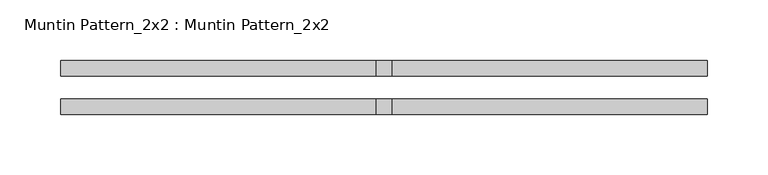
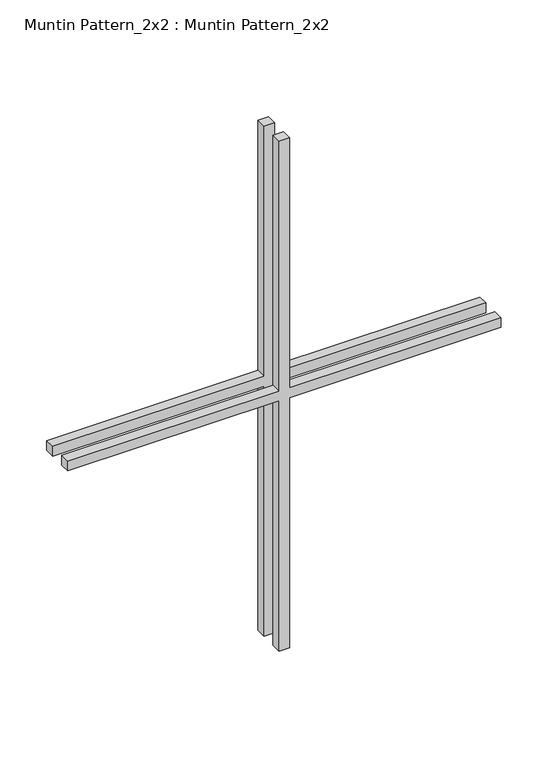
"""IFC4 building model written with IfcOpenShell, lengths in millimetres: proxy geometry, Muntin Pattern_2x2 : Muntin Pattern_2x2."""

from ifc_helpers import new_model, si_unit, frame, origin, place, context, project, spatial, polyline, outline, extrude, source, transform, mapped, element, save


def muntin_pattern_2x2_muntin_pattern_2x2_f10761d2(model_context):
    return source(origin(), model_context, "Body", "SweptSolid", [
        extrude(outline(polyline([(338.1375, -6.35), (338.1375, -266.7), (325.4375, -266.7), (325.4375, -6.35), (0.0, -6.35), (0.0, 6.35), (325.4375, 6.35), (325.4375, 266.7), (338.1375, 266.7), (338.1375, 6.35), (663.575, 6.35), (663.575, -6.35), (338.1375, -6.35)])), frame((0.0, -22.225, 0.0), z_axis=(0.0, 1.0, 0.0), x_axis=(0.0, 0.0, 1.0)), (0.0, 0.0, 1.0), 12.7),
        extrude(outline(polyline([(338.1375, -6.35), (338.1375, -266.7), (325.4375, -266.7), (325.4375, -6.35), (0.0, -6.35), (0.0, 6.35), (325.4375, 6.35), (325.4375, 266.7), (338.1375, 266.7), (338.1375, 6.35), (663.575, 6.35), (663.575, -6.35), (338.1375, -6.35)])), frame((0.0, 9.525, 0.0), z_axis=(0.0, 1.0, 0.0), x_axis=(0.0, 0.0, 1.0)), (0.0, 0.0, 1.0), 12.7),
    ])


if __name__ == "__main__":
    model = new_model("IFC4")
    model_context = context("Model", 3, world=origin())
    ifc_project = project(units=[si_unit("LENGTHUNIT", "METRE", prefix="MILLI")], contexts=[model_context])
    site = spatial("IfcSite", under=ifc_project)
    building = spatial("IfcBuilding", under=site)
    placement = place(None, origin())
    muntin_pattern_2x2_muntin_pattern_2x2_shape = muntin_pattern_2x2_muntin_pattern_2x2_f10761d2(model_context)
    element("IfcBuildingElementProxy", 1, Name="Muntin Pattern_2x2 : Muntin Pattern_2x2", ObjectType="Muntin Pattern_2x2 : Muntin Pattern_2x2", at=placement, inside=building, context=model_context, shape_type="MappedRepresentation", body=[
        mapped(muntin_pattern_2x2_muntin_pattern_2x2_shape, transform((0.0, 0.0, 0.0), x_axis=(1.0, 0.0, 0.0), y_axis=(0.0, 1.0, 0.0), z_axis=(0.0, 0.0, 1.0))),
    ])
    save(model, "model.ifc")

# Revit data of these elements
# Type "Muntin Pattern_2x2 : Muntin Pattern_2x2"
#   Width [instance default] = 4' - 0"
#   Thickness = 0' - 0 1/2"
#   Height [instance default] = 4' - 0"
#   Distance = 0' - 0 3/4"
#   Interior Material [instance default] = none
#   Exterior Material [instance default] = none
#   Default Elevation = 0
# Element 1 (IfcBuildingElementProxy, "Muntin Pattern_2x2 : Muntin Pattern_2x2")
#   Width = 1' - 9"
#   Height = 2' - 2 1/8"
#   Interior Material = Wood - Stained
#   Exterior Material = Clad - White
#   Materials on its faces: "Clad - White", "Wood - Stained"
# Materials
#   "Clad - White": class "Wood", colour RGB 242 242 238, transparency 0, Cost = 0
#   "Wood - Stained": class "Wood", colour RGB 224 178 126, transparency 0, Cost = 0
